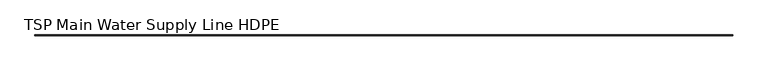
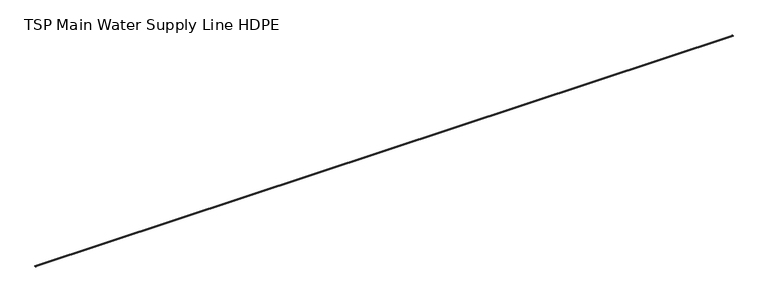
"""IFC4 building model written with IfcOpenShell, lengths in millimetres: flow terminal geometry, TSP Main Water Supply Line HDPE : HDPE Fresh Water Supply."""

import ifcopenshell
import ifcopenshell.guid

model = None  # the IFC model being written
_history = None  # IfcOwnerHistory: only IFC2X3 demands one
_inside = {}  # id of a spatial element -> (the spatial element, [elements in it])
_under = {}  # id of a project, library or spatial element -> (it, [spatial elements below it])
_declared = {}  # id of a project -> (the project, [libraries it declares])
_typed = {}  # id of a type object -> (the type object, [elements of that type])
_made_of = {}  # id of a material, layer set ... -> (it, [elements and type objects made of it])


def new_model(schema):
    """Start an empty IFC model of exactly this schema.

    Asked for "IFC4X3", IfcOpenShell would pick the latest addendum, in which some entities
    have other attributes; the version numbers below select the first issue.
    IFC2X3 requires an IfcOwnerHistory on every rooted entity: one is made here for all.
    """
    global model, _history
    if schema == "IFC4X3":
        model = ifcopenshell.file(schema_version=(4, 3, 0, 0))
    else:
        model = ifcopenshell.file(schema=schema)
    _inside.clear()
    _under.clear()
    _declared.clear()
    _typed.clear()
    _made_of.clear()
    _history = None
    if model.schema == "IFC2X3":
        org = make("IfcOrganization", Name="unknown")
        user = make(
            "IfcPersonAndOrganization",
            ThePerson=make("IfcPerson", FamilyName="unknown"),
            TheOrganization=org,
        )
        app = make(
            "IfcApplication",
            ApplicationDeveloper=org,
            Version="unknown",
            ApplicationFullName="unknown",
            ApplicationIdentifier="unknown",
        )
        _history = make(
            "IfcOwnerHistory",
            OwningUser=user,
            OwningApplication=app,
            ChangeAction="ADDED",
            CreationDate=0,
        )
    return model


def make(cls, **values):
    """One entity of the class cls with the attributes given. An attribute that is None is left unset."""
    return model.create_entity(
        cls, **{name: value for name, value in values.items() if value is not None}
    )


def rooted(cls, **values):
    """An entity with a GlobalId (a new one), such as an element, a storey or a relation."""
    return make(cls, GlobalId=ifcopenshell.guid.new(), OwnerHistory=_history, **values)


def si_unit(unit_type, name, prefix=None):
    """IfcSIUnit, for example si_unit("LENGTHUNIT", "METRE", prefix="MILLI")."""
    return make("IfcSIUnit", UnitType=unit_type, Prefix=prefix, Name=name)


def assignment(units):
    """IfcUnitAssignment: the units of a project."""
    return None if units is None else make("IfcUnitAssignment", Units=units)


def point(xyz):
    """IfcCartesianPoint."""
    return None if xyz is None else make("IfcCartesianPoint", Coordinates=xyz)


def direction(xyz):
    """IfcDirection."""
    return None if xyz is None else make("IfcDirection", DirectionRatios=xyz)


def frame(location, z_axis=None, x_axis=None):
    """IfcAxis2Placement3D, a coordinate frame: its origin and axes. An axis left out is left unset."""
    return make(
        "IfcAxis2Placement3D",
        Location=point(location),
        Axis=direction(z_axis),
        RefDirection=direction(x_axis),
    )


def frame_2d(location, x_axis=None):
    """IfcAxis2Placement2D, a coordinate frame in the plane: its origin and x axis."""
    return make(
        "IfcAxis2Placement2D", Location=point(location), RefDirection=direction(x_axis)
    )


def origin():
    """The frame at (0, 0, 0) with its axes left unset."""
    return frame((0.0, 0.0, 0.0))


def origin_2d():
    """The frame at (0, 0) in the plane with its x axis left unset."""
    return frame_2d((0.0, 0.0))


def place(relative_to, where):
    """IfcLocalPlacement: puts the frame where relative to a parent placement (None: the world)."""
    return make(
        "IfcLocalPlacement", PlacementRelTo=relative_to, RelativePlacement=where
    )


def context(
    kind, dimensions, precision=None, world=None, true_north=None, identifier=None
):
    """IfcGeometricRepresentationContext, for example the 3D "Model" context."""
    return make(
        "IfcGeometricRepresentationContext",
        ContextIdentifier=identifier,
        ContextType=kind,
        CoordinateSpaceDimension=dimensions,
        Precision=precision,
        WorldCoordinateSystem=world,
        TrueNorth=true_north,
    )


def project(units=None, contexts=None):
    """IfcProject with its units and contexts."""
    return rooted(
        "IfcProject",
        Name="project",
        RepresentationContexts=contexts,
        UnitsInContext=assignment(units),
    )


def spatial(cls, under=None, at=None, **own):
    """A site, building, storey or space (cls), placed at a placement, below another one or the project."""
    s = rooted(cls, ObjectPlacement=at, **own)
    if under is not None:
        _under.setdefault(under.id(), (under, []))[1].append(s)
    return s


def circle_curve(where, radius):
    """IfcCircle in the frame where."""
    return make("IfcCircle", Position=where, Radius=radius)


def trimmed(basis, trim1, trim2, sense, master):
    """IfcTrimmedCurve: the piece of a basis curve between two trims."""
    return make(
        "IfcTrimmedCurve",
        BasisCurve=basis,
        Trim1=trim1,
        Trim2=trim2,
        SenseAgreement=sense,
        MasterRepresentation=master,
    )


def segment(curve, same_sense, transition):
    """IfcCompositeCurveSegment."""
    return make(
        "IfcCompositeCurveSegment",
        Transition=transition,
        SameSense=same_sense,
        ParentCurve=curve,
    )


def composite_curve(segments, self_intersect=None):
    """IfcCompositeCurve: segments joined end to end."""
    return make("IfcCompositeCurve", Segments=segments, SelfIntersect=self_intersect)


def outline(outer, holes=None, kind="AREA"):
    """IfcArbitraryClosedProfileDef: a profile drawn as a closed curve; with holes, ...WithVoids."""
    if holes is None:
        return make("IfcArbitraryClosedProfileDef", ProfileType=kind, OuterCurve=outer)
    return make(
        "IfcArbitraryProfileDefWithVoids",
        ProfileType=kind,
        OuterCurve=outer,
        InnerCurves=holes,
    )


def extrude(swept, where, along, depth):
    """IfcExtrudedAreaSolid: the profile swept, set in the frame where, extruded along a direction by depth."""
    return make(
        "IfcExtrudedAreaSolid",
        SweptArea=swept,
        Position=where,
        ExtrudedDirection=direction(along),
        Depth=depth,
    )


def shape(context_of_items, identifier, shape_type, items):
    """IfcShapeRepresentation: the items that make up one representation, for example the "Body"."""
    return make(
        "IfcShapeRepresentation",
        ContextOfItems=context_of_items,
        RepresentationIdentifier=identifier,
        RepresentationType=shape_type,
        Items=items,
    )


def source(mapping_origin, context_of_items, identifier, shape_type, items):
    """IfcRepresentationMap: a shape defined once, which mapped items show again and again."""
    return make(
        "IfcRepresentationMap",
        MappingOrigin=mapping_origin,
        MappedRepresentation=shape(context_of_items, identifier, shape_type, items),
    )


def transform(
    local_origin,
    x_axis=None,
    y_axis=None,
    z_axis=None,
    scale=None,
    scale2=None,
    scale3=None,
    uniform=True,
):
    """IfcCartesianTransformationOperator3D, or its non-uniform kind. x_axis, y_axis, z_axis: its Axis1, 2, 3."""
    if uniform:
        return make(
            "IfcCartesianTransformationOperator3D",
            Axis1=direction(x_axis),
            Axis2=direction(y_axis),
            LocalOrigin=point(local_origin),
            Scale=scale,
            Axis3=direction(z_axis),
        )
    return make(
        "IfcCartesianTransformationOperator3DnonUniform",
        Axis1=direction(x_axis),
        Axis2=direction(y_axis),
        LocalOrigin=point(local_origin),
        Scale=scale,
        Axis3=direction(z_axis),
        Scale2=scale2,
        Scale3=scale3,
    )


def mapped(mapping_source, mapping_target):
    """IfcMappedItem: shows the shape of a source again, moved by a transform."""
    return make(
        "IfcMappedItem", MappingSource=mapping_source, MappingTarget=mapping_target
    )


def made_of(thing, what):
    """Note that an element or type object is made of a material, layer set ...; save() writes the relation."""
    if what is not None:
        _made_of.setdefault(what.id(), (what, []))[1].append(thing)
    return thing


def element(
    cls,
    number,
    at=None,
    inside=None,
    cuts=None,
    type_object=None,
    material=None,
    context=None,
    identifier="Body",
    shape_type=None,
    held_by="IfcProductDefinitionShape",
    body=None,
    shapes=None,
    **own,
):
    """One element of the class cls, such as IfcWall. Its Tag is "e" and its number.

    at: its placement. inside: the storey or other place that contains it. cuts: it is an
    opening in that element (IfcRelVoidsElement). A single representation is given by context,
    identifier, shape_type and body (its items); several are given by shapes. held_by: the class
    of the entity that holds the representations. save() writes the other relations.
    """
    e = rooted(cls, Tag="e%d" % number, ObjectPlacement=at, **own)
    if body is not None:
        shapes = [shape(context, identifier, shape_type, body)]
    if shapes is not None:
        e.Representation = make(held_by, Representations=shapes)
    if inside is not None:
        _inside.setdefault(inside.id(), (inside, []))[1].append(e)
    if cuts is not None:
        rooted(
            "IfcRelVoidsElement", RelatingBuildingElement=cuts, RelatedOpeningElement=e
        )
    if type_object is not None:
        _typed.setdefault(type_object.id(), (type_object, []))[1].append(e)
    return made_of(e, material)


def aggregate(whole, parts):
    """IfcRelAggregates: a whole, such as a stair, and the parts it consists of."""
    return rooted("IfcRelAggregates", RelatingObject=whole, RelatedObjects=parts)


def save(model, path):
    """Write the relations noted so far, then the file.

    IfcRelAggregates (storeys below a building ...), IfcRelContainedInSpatialStructure (elements
    in a storey), IfcRelDefinesByType, IfcRelAssociatesMaterial and IfcRelDeclares: one each for
    every whole, place, type object, material and project.
    """
    for whole, parts in _under.values():
        aggregate(whole, parts)
    for where, things in _inside.values():
        rooted(
            "IfcRelContainedInSpatialStructure",
            RelatedElements=things,
            RelatingStructure=where,
        )
    for kind, things in _typed.values():
        rooted("IfcRelDefinesByType", RelatedObjects=things, RelatingType=kind)
    for what, things in _made_of.values():
        rooted("IfcRelAssociatesMaterial", RelatedObjects=things, RelatingMaterial=what)
    for by, libraries in _declared.values():
        rooted("IfcRelDeclares", RelatingContext=by, RelatedDefinitions=libraries)
    model.write(path)


def tsp_main_water_supply_line_hdpe_8955a997(model_context):
    return source(origin(), model_context, "Body", "SweptSolid", [
        extrude(outline(composite_curve([segment(trimmed(circle_curve(origin_2d(), 16.0), [point((-16.0, 0.0))], [point((16.0, 0.0))], False, "CARTESIAN"), True, "CONTINUOUS"), segment(trimmed(circle_curve(origin_2d(), 16.0), [point((16.0, 0.0))], [point((-16.0, 0.0))], False, "CARTESIAN"), True, "CONTINUOUS")], self_intersect=False), holes=[composite_curve([segment(trimmed(circle_curve(origin_2d(), 15.0), [point((-15.0, 0.0))], [point((15.0, 0.0))], True, "CARTESIAN"), True, "CONTINUOUS"), segment(trimmed(circle_curve(origin_2d(), 15.0), [point((15.0, 0.0))], [point((-15.0, 0.0))], True, "CARTESIAN"), True, "CONTINUOUS")], self_intersect=False)]), frame((0.0, 0.0, 0.0), z_axis=(1.0, 0.0, 0.0), x_axis=(0.0, 1.0, 0.0)), (0.0, 0.0, 1.0), 21857.8141272),
    ])


if __name__ == "__main__":
    model = new_model("IFC4")
    model_context = context("Model", 3, world=origin())
    ifc_project = project(units=[si_unit("LENGTHUNIT", "METRE", prefix="MILLI")], contexts=[model_context])
    site = spatial("IfcSite", under=ifc_project)
    building = spatial("IfcBuilding", under=site)
    placement = place(None, origin())
    tsp_main_water_supply_line_hdpe_shape = tsp_main_water_supply_line_hdpe_8955a997(model_context)
    element("IfcFlowTerminal", 1, ObjectType="TSP Main Water Supply Line HDPE : HDPE Fresh Water Supply", at=placement, inside=building, context=model_context, shape_type="MappedRepresentation", body=[
        mapped(tsp_main_water_supply_line_hdpe_shape, transform((0.0, 0.0, 0.0), x_axis=(1.0, 0.0, 0.0), y_axis=(0.0, 1.0, 0.0), z_axis=(0.0, 0.0, 1.0))),
    ])
    save(model, "model.ifc")

# Revit data of these elements
# Type "TSP Main Water Supply Line HDPE : HDPE Fresh Water Supply"
#   Model = "TSP_110SFWSP"
#   Pipe length [instance default] = 1200 mm
#   Pipe dia = 30 mm
#   built-in parameter 1001306 [instance default] = 3.93701 (stored number, unit not read)
#   Default Elevation = 0
# Element 1 (IfcFlowTerminal, "TSP Main Water Supply Line HDPE : HDPE Fresh Water Supply")
#   Pipe length = 21857.814 mm
#   built-in parameter 1001306 = 71.712 (stored number, unit not read)
#   Materials on its faces: "Aluminum, Anodized Blue"
# Materials
#   "Aluminum, Anodized Blue": class "Metal", colour RGB 120 120 120, transparency 0, Description = "Anodized aluminum, blue", Cost = 0
